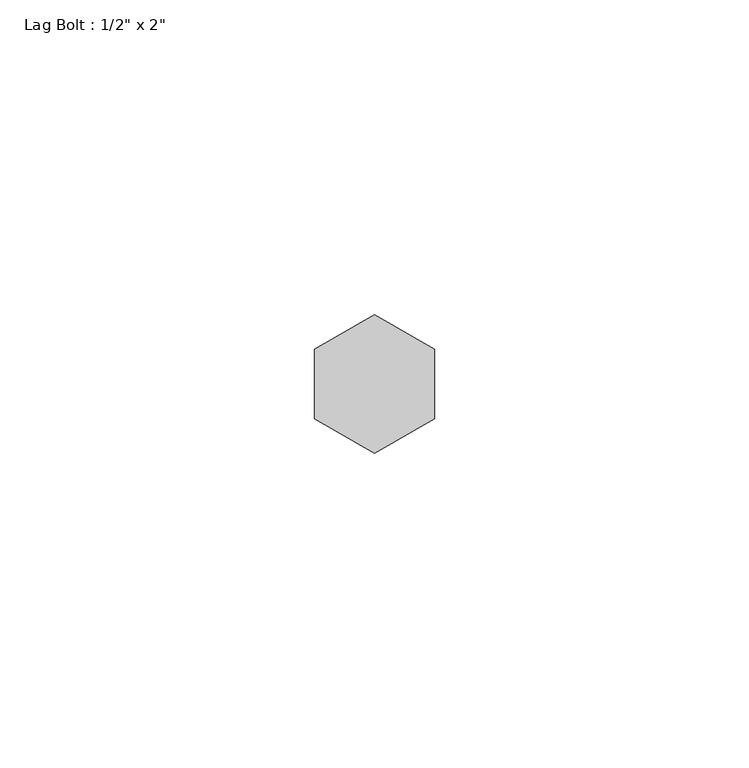
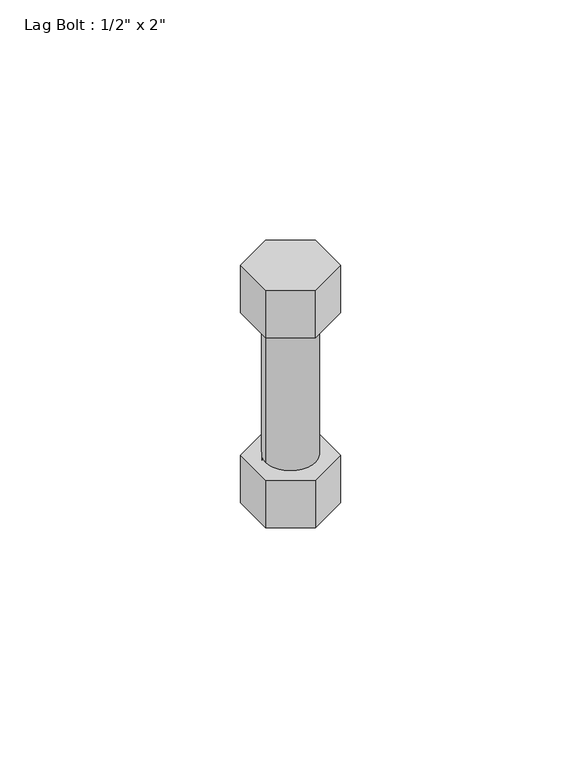
"""IFC4 building model written with IfcOpenShell, lengths in millimetres: proxy geometry."""

from ifc_helpers import new_model, si_unit, point, frame, origin, origin_with_axes, origin_2d, place, context, project, spatial, polyline, circle_curve, trimmed, segment, composite_curve, outline, extrude, source, transform, mapped, element, save


def proxy_30a1c0d9(model_context):
    return source(origin(), model_context, "Body", "SweptSolid", [
        extrude(outline(polyline([(-9.525, 5.4992613), (0.0, 10.9985226), (9.525, 5.4992613), (9.525, -5.4992613), (0.0, -10.9985226), (-9.525, -5.4992613), (-9.525, 5.4992613)])), frame((0.0, 0.0, -50.8), z_axis=(0.0, 0.0, 1.0), x_axis=(1.0, 0.0, 0.0)), (0.0, 0.0, 1.0), 12.7),
        extrude(outline(polyline([(-9.525, -5.4992613), (-9.525, 5.4992613), (0.0, 10.9985226), (9.525, 5.4992613), (9.525, -5.4992613), (0.0, -10.9985226), (-9.525, -5.4992613)])), origin_with_axes(), (0.0, 0.0, 1.0), 12.7),
        extrude(outline(composite_curve([segment(trimmed(circle_curve(origin_2d(), 6.35), [point((-6.35, 0.0))], [point((6.35, 0.0))], False, "CARTESIAN"), True, "CONTINUOUS"), segment(trimmed(circle_curve(origin_2d(), 6.35), [point((6.35, 0.0))], [point((-6.35, 0.0))], False, "CARTESIAN"), True, "CONTINUOUS")], self_intersect=False)), frame((0.0, 0.0, -50.8), z_axis=(0.0, 0.0, 1.0), x_axis=(1.0, 0.0, 0.0)), (0.0, 0.0, 1.0), 50.8),
    ])


if __name__ == "__main__":
    model = new_model("IFC4")
    model_context = context("Model", 3, world=origin())
    ifc_project = project(units=[si_unit("LENGTHUNIT", "METRE", prefix="MILLI")], contexts=[model_context])
    site = spatial("IfcSite", under=ifc_project)
    building = spatial("IfcBuilding", under=site)
    placement = place(None, origin())
    proxy_shape = proxy_30a1c0d9(model_context)
    element("IfcBuildingElementProxy", 1, Name="Lag Bolt : 1/2\" x 2\"", ObjectType="Lag Bolt : 1/2\" x 2\"", at=placement, inside=building, context=model_context, shape_type="MappedRepresentation", body=[
        mapped(proxy_shape, transform((0.0, 0.0, 0.0), x_axis=(1.0, 0.0, 0.0), y_axis=(0.0, 1.0, 0.0), z_axis=(0.0, 0.0, 1.0))),
    ])
    save(model, "model.ifc")

# Revit data of these elements
# Type "Lag Bolt : 1/2\" x 2\""
#   Thickness_of_Substrate [instance default] = 0' - 1"
#   Side = 0' - 0 111/256"
#   Radius = 0' - 0 1/4"
#   Length = 0' - 2"
#   Head Size = 0' - 0 3/4"
#   Head Radius = 0' - 0 3/8"
#   Head Height = 0' - 0 1/2"
#   Diameter = 0' - 0 1/2"
#   Default Elevation = 4' - 0"
#   Nut_Visibility [instance default] = yes
#   Bolt Material (Size) [instance default] = 1" GALV. LAG BOLT (LENGTH = 1/2" SHY OF GLULAM DEPTH) -  (GALV. THRU BOLT IF PLATE ON OPP. SIDE OF STRUCT MEMBER)
# Element 1 (IfcBuildingElementProxy, "Lag Bolt : 1/2\" x 2\"")
#   Thickness_of_Substrate = 0' - 1 1/2"
#   Bolt Material (Size) = 1/2 LAG BOLTS 24" O.C.
#   Materials on its faces: "1/2 LAG BOLTS 24\" O.C.", "STRUCTURAL BOLTS (PAINT TO MATCH STEEL FINISH)"
# Materials
#   "1\" GALV. LAG BOLT (LENGTH = 1/2\" SHY OF GLULAM DEPTH) -  (GALV. THRU BOLT IF PLATE ON OPP. SIDE OF STRUCT MEMBER)": class "Generic", colour RGB 120 120 120, transparency 0, Cost = 0
#   "1/2 LAG BOLTS 24\" O.C.": class "Generic", colour RGB 120 120 120, transparency 0, Cost = 0
#   "STRUCTURAL BOLTS (PAINT TO MATCH STEEL FINISH)": class "Generic", colour RGB 120 120 120, transparency 0, Cost = 0
